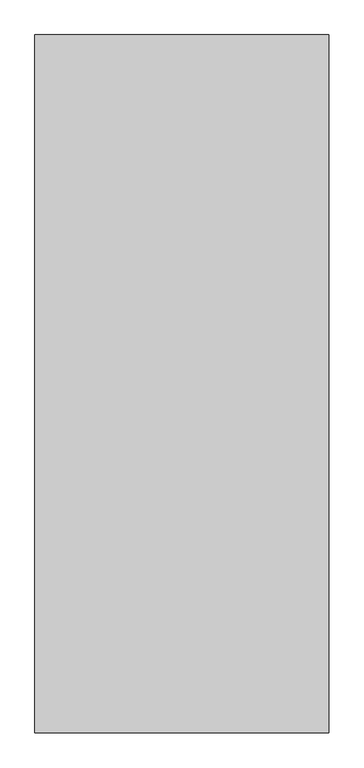
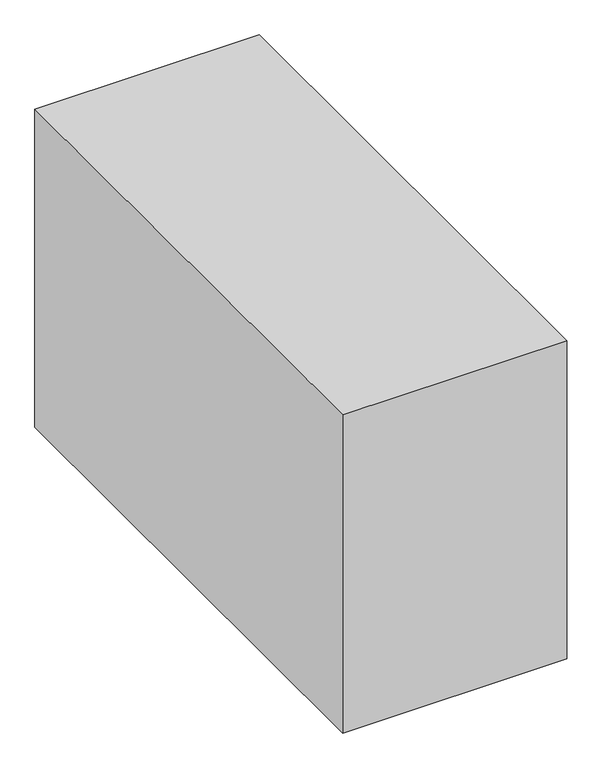
"""IFC4 building model written with IfcOpenShell, lengths in millimetres: proxy geometry, Space Planning Box_hec : Space Planning Box_hec."""

import ifcopenshell
import ifcopenshell.guid

model = None  # the IFC model being written
_history = None  # IfcOwnerHistory: only IFC2X3 demands one
_inside = {}  # id of a spatial element -> (the spatial element, [elements in it])
_under = {}  # id of a project, library or spatial element -> (it, [spatial elements below it])
_declared = {}  # id of a project -> (the project, [libraries it declares])
_typed = {}  # id of a type object -> (the type object, [elements of that type])
_made_of = {}  # id of a material, layer set ... -> (it, [elements and type objects made of it])


def new_model(schema):
    """Start an empty IFC model of exactly this schema.

    Asked for "IFC4X3", IfcOpenShell would pick the latest addendum, in which some entities
    have other attributes; the version numbers below select the first issue.
    IFC2X3 requires an IfcOwnerHistory on every rooted entity: one is made here for all.
    """
    global model, _history
    if schema == "IFC4X3":
        model = ifcopenshell.file(schema_version=(4, 3, 0, 0))
    else:
        model = ifcopenshell.file(schema=schema)
    _inside.clear()
    _under.clear()
    _declared.clear()
    _typed.clear()
    _made_of.clear()
    _history = None
    if model.schema == "IFC2X3":
        org = make("IfcOrganization", Name="unknown")
        user = make(
            "IfcPersonAndOrganization",
            ThePerson=make("IfcPerson", FamilyName="unknown"),
            TheOrganization=org,
        )
        app = make(
            "IfcApplication",
            ApplicationDeveloper=org,
            Version="unknown",
            ApplicationFullName="unknown",
            ApplicationIdentifier="unknown",
        )
        _history = make(
            "IfcOwnerHistory",
            OwningUser=user,
            OwningApplication=app,
            ChangeAction="ADDED",
            CreationDate=0,
        )
    return model


def make(cls, **values):
    """One entity of the class cls with the attributes given. An attribute that is None is left unset."""
    return model.create_entity(
        cls, **{name: value for name, value in values.items() if value is not None}
    )


def rooted(cls, **values):
    """An entity with a GlobalId (a new one), such as an element, a storey or a relation."""
    return make(cls, GlobalId=ifcopenshell.guid.new(), OwnerHistory=_history, **values)


def si_unit(unit_type, name, prefix=None):
    """IfcSIUnit, for example si_unit("LENGTHUNIT", "METRE", prefix="MILLI")."""
    return make("IfcSIUnit", UnitType=unit_type, Prefix=prefix, Name=name)


def assignment(units):
    """IfcUnitAssignment: the units of a project."""
    return None if units is None else make("IfcUnitAssignment", Units=units)


def point(xyz):
    """IfcCartesianPoint."""
    return None if xyz is None else make("IfcCartesianPoint", Coordinates=xyz)


def direction(xyz):
    """IfcDirection."""
    return None if xyz is None else make("IfcDirection", DirectionRatios=xyz)


def frame(location, z_axis=None, x_axis=None):
    """IfcAxis2Placement3D, a coordinate frame: its origin and axes. An axis left out is left unset."""
    return make(
        "IfcAxis2Placement3D",
        Location=point(location),
        Axis=direction(z_axis),
        RefDirection=direction(x_axis),
    )


def origin():
    """The frame at (0, 0, 0) with its axes left unset."""
    return frame((0.0, 0.0, 0.0))


def origin_with_axes():
    """The frame at (0, 0, 0) with the z axis (0, 0, 1) and the x axis (1, 0, 0) written out."""
    return frame((0.0, 0.0, 0.0), z_axis=(0.0, 0.0, 1.0), x_axis=(1.0, 0.0, 0.0))


def place(relative_to, where):
    """IfcLocalPlacement: puts the frame where relative to a parent placement (None: the world)."""
    return make(
        "IfcLocalPlacement", PlacementRelTo=relative_to, RelativePlacement=where
    )


def context(
    kind, dimensions, precision=None, world=None, true_north=None, identifier=None
):
    """IfcGeometricRepresentationContext, for example the 3D "Model" context."""
    return make(
        "IfcGeometricRepresentationContext",
        ContextIdentifier=identifier,
        ContextType=kind,
        CoordinateSpaceDimension=dimensions,
        Precision=precision,
        WorldCoordinateSystem=world,
        TrueNorth=true_north,
    )


def project(units=None, contexts=None):
    """IfcProject with its units and contexts."""
    return rooted(
        "IfcProject",
        Name="project",
        RepresentationContexts=contexts,
        UnitsInContext=assignment(units),
    )


def spatial(cls, under=None, at=None, **own):
    """A site, building, storey or space (cls), placed at a placement, below another one or the project."""
    s = rooted(cls, ObjectPlacement=at, **own)
    if under is not None:
        _under.setdefault(under.id(), (under, []))[1].append(s)
    return s


def polyline(points):
    """IfcPolyline through the points."""
    return make("IfcPolyline", Points=[point(p) for p in points])


def outline(outer, holes=None, kind="AREA"):
    """IfcArbitraryClosedProfileDef: a profile drawn as a closed curve; with holes, ...WithVoids."""
    if holes is None:
        return make("IfcArbitraryClosedProfileDef", ProfileType=kind, OuterCurve=outer)
    return make(
        "IfcArbitraryProfileDefWithVoids",
        ProfileType=kind,
        OuterCurve=outer,
        InnerCurves=holes,
    )


def extrude(swept, where, along, depth):
    """IfcExtrudedAreaSolid: the profile swept, set in the frame where, extruded along a direction by depth."""
    return make(
        "IfcExtrudedAreaSolid",
        SweptArea=swept,
        Position=where,
        ExtrudedDirection=direction(along),
        Depth=depth,
    )


def shape(context_of_items, identifier, shape_type, items):
    """IfcShapeRepresentation: the items that make up one representation, for example the "Body"."""
    return make(
        "IfcShapeRepresentation",
        ContextOfItems=context_of_items,
        RepresentationIdentifier=identifier,
        RepresentationType=shape_type,
        Items=items,
    )


def source(mapping_origin, context_of_items, identifier, shape_type, items):
    """IfcRepresentationMap: a shape defined once, which mapped items show again and again."""
    return make(
        "IfcRepresentationMap",
        MappingOrigin=mapping_origin,
        MappedRepresentation=shape(context_of_items, identifier, shape_type, items),
    )


def transform(
    local_origin,
    x_axis=None,
    y_axis=None,
    z_axis=None,
    scale=None,
    scale2=None,
    scale3=None,
    uniform=True,
):
    """IfcCartesianTransformationOperator3D, or its non-uniform kind. x_axis, y_axis, z_axis: its Axis1, 2, 3."""
    if uniform:
        return make(
            "IfcCartesianTransformationOperator3D",
            Axis1=direction(x_axis),
            Axis2=direction(y_axis),
            LocalOrigin=point(local_origin),
            Scale=scale,
            Axis3=direction(z_axis),
        )
    return make(
        "IfcCartesianTransformationOperator3DnonUniform",
        Axis1=direction(x_axis),
        Axis2=direction(y_axis),
        LocalOrigin=point(local_origin),
        Scale=scale,
        Axis3=direction(z_axis),
        Scale2=scale2,
        Scale3=scale3,
    )


def mapped(mapping_source, mapping_target):
    """IfcMappedItem: shows the shape of a source again, moved by a transform."""
    return make(
        "IfcMappedItem", MappingSource=mapping_source, MappingTarget=mapping_target
    )


def made_of(thing, what):
    """Note that an element or type object is made of a material, layer set ...; save() writes the relation."""
    if what is not None:
        _made_of.setdefault(what.id(), (what, []))[1].append(thing)
    return thing


def element(
    cls,
    number,
    at=None,
    inside=None,
    cuts=None,
    type_object=None,
    material=None,
    context=None,
    identifier="Body",
    shape_type=None,
    held_by="IfcProductDefinitionShape",
    body=None,
    shapes=None,
    **own,
):
    """One element of the class cls, such as IfcWall. Its Tag is "e" and its number.

    at: its placement. inside: the storey or other place that contains it. cuts: it is an
    opening in that element (IfcRelVoidsElement). A single representation is given by context,
    identifier, shape_type and body (its items); several are given by shapes. held_by: the class
    of the entity that holds the representations. save() writes the other relations.
    """
    e = rooted(cls, Tag="e%d" % number, ObjectPlacement=at, **own)
    if body is not None:
        shapes = [shape(context, identifier, shape_type, body)]
    if shapes is not None:
        e.Representation = make(held_by, Representations=shapes)
    if inside is not None:
        _inside.setdefault(inside.id(), (inside, []))[1].append(e)
    if cuts is not None:
        rooted(
            "IfcRelVoidsElement", RelatingBuildingElement=cuts, RelatedOpeningElement=e
        )
    if type_object is not None:
        _typed.setdefault(type_object.id(), (type_object, []))[1].append(e)
    return made_of(e, material)


def aggregate(whole, parts):
    """IfcRelAggregates: a whole, such as a stair, and the parts it consists of."""
    return rooted("IfcRelAggregates", RelatingObject=whole, RelatedObjects=parts)


def save(model, path):
    """Write the relations noted so far, then the file.

    IfcRelAggregates (storeys below a building ...), IfcRelContainedInSpatialStructure (elements
    in a storey), IfcRelDefinesByType, IfcRelAssociatesMaterial and IfcRelDeclares: one each for
    every whole, place, type object, material and project.
    """
    for whole, parts in _under.values():
        aggregate(whole, parts)
    for where, things in _inside.values():
        rooted(
            "IfcRelContainedInSpatialStructure",
            RelatedElements=things,
            RelatingStructure=where,
        )
    for kind, things in _typed.values():
        rooted("IfcRelDefinesByType", RelatedObjects=things, RelatingType=kind)
    for what, things in _made_of.values():
        rooted("IfcRelAssociatesMaterial", RelatedObjects=things, RelatingMaterial=what)
    for by, libraries in _declared.values():
        rooted("IfcRelDeclares", RelatingContext=by, RelatedDefinitions=libraries)
    model.write(path)


def generic_models_3a820573(model_context):
    return source(origin(), model_context, "Body", "SweptSolid", [
        extrude(outline(polyline([(2000.0, 4750.0), (2000.0, -4750.0), (-2000.0, -4750.0), (-2000.0, 4750.0), (2000.0, 4750.0)])), origin_with_axes(), (0.0, 0.0, 1.0), 6000.0),
    ])


if __name__ == "__main__":
    model = new_model("IFC4")
    model_context = context("Model", 3, world=origin())
    ifc_project = project(units=[si_unit("LENGTHUNIT", "METRE", prefix="MILLI")], contexts=[model_context])
    site = spatial("IfcSite", under=ifc_project)
    building = spatial("IfcBuilding", under=site)
    placement = place(None, origin())
    generic_models_shape = generic_models_3a820573(model_context)
    element("IfcBuildingElementProxy", 1, Name="Space Planning Box_hec : Space Planning Box_hec", ObjectType="Space Planning Box_hec : Space Planning Box_hec", at=placement, inside=building, context=model_context, shape_type="MappedRepresentation", body=[
        mapped(generic_models_shape, transform((0.0, 0.0, 0.0), x_axis=(1.0, 0.0, 0.0), y_axis=(0.0, 1.0, 0.0), z_axis=(0.0, 0.0, 1.0))),
    ])
    save(model, "model.ifc")

# Revit data of these elements
# Type "Space Planning Box_hec : Space Planning Box_hec"
#   Type Comments = "..."
#   Room Name [instance default] = "?"
#   Interior Finish [instance default] = ""
#   Exterior Finish [instance default] = ""
#   Department [instance default] = ""
#   Assembly Code = "..."
#   Width [instance default] = 1524 mm
#   Program Area [instance default] = 0.00 m²
#   Length [instance default] = 1524 mm
#   Height [instance default] = 1524 mm
#   Area [instance default] = 2.32258 m²
#   Fill Color [instance default] = Cyan
#   Default Elevation = 0
# Element 1 (IfcBuildingElementProxy, "Space Planning Box_hec : Space Planning Box_hec")
#   Room Name = "Stairway"
#   Interior Finish = "IF2"
#   Exterior Finish = "EF1"
#   Department = "AR"
#   Width = 4000 mm
#   Program Area = 38.00 m²
#   Length = 9500 mm
#   Height = 6000 mm
#   Area = 38.00 m²
#   Fill Color = Lavender
#   Materials on its faces: "Lavender"
# Materials
#   "Cyan": class "Generic", colour RGB 0 255 255, transparency 0.2, Cost = 0
#   "Lavender": class "Generic", colour RGB 186 85 211, transparency 0.2, Cost = 0
